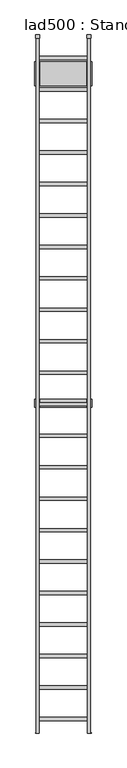
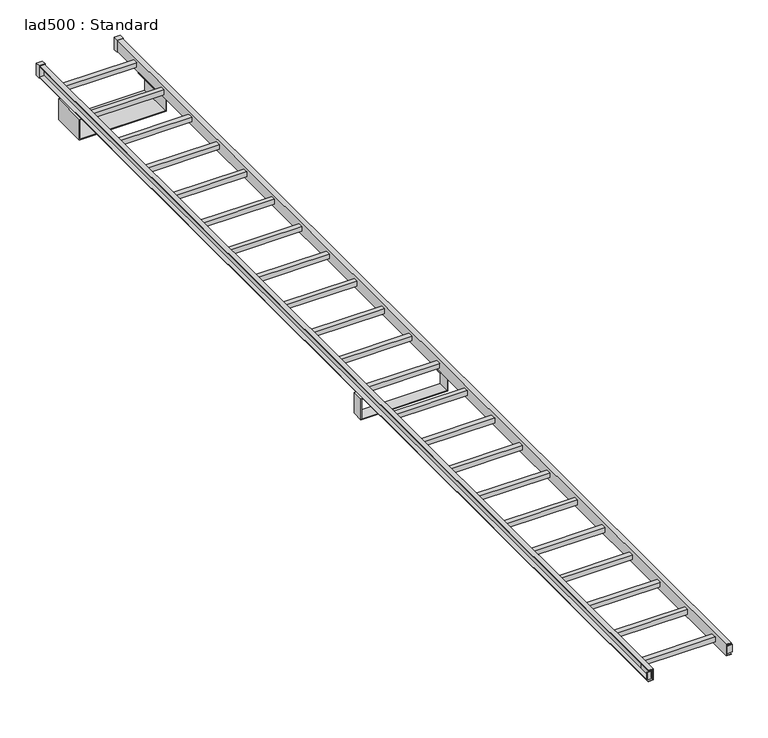
"""IFC4 building model written with IfcOpenShell, lengths in millimetres: proxy geometry, lad500 : Standard."""

from ifc_helpers import new_model, si_unit, point, frame, frame_2d, origin, place, context, project, spatial, polyline, circle_curve, trimmed, segment, composite_curve, outline, extrude, source, transform, mapped, element, save


def lad500_standard_3a90afe1(model_context):
    return source(origin(), model_context, "Body", "SweptSolid", [
        extrude(outline(polyline([(-233.3625, -1309.5859108), (-233.3625, -1277.8359108), (233.3625, -1277.8359108), (233.3625, -1309.5859108), (-233.3625, -1309.5859108)])), frame((0.0, 0.0, 161.925), z_axis=(0.0, 0.0, 1.0), x_axis=(1.0, 0.0, 0.0)), (0.0, 0.0, 1.0), 31.75),
        extrude(outline(polyline([(-233.3625, -1004.7859108), (-233.3625, -973.0359108), (233.3625, -973.0359108), (233.3625, -1004.7859108), (-233.3625, -1004.7859108)])), frame((0.0, 0.0, 161.925), z_axis=(0.0, 0.0, 1.0), x_axis=(1.0, 0.0, 0.0)), (0.0, 0.0, 1.0), 31.75),
        extrude(outline(polyline([(-233.3625, -699.9859108), (-233.3625, -668.2359108), (233.3625, -668.2359108), (233.3625, -699.9859108), (-233.3625, -699.9859108)])), frame((0.0, 0.0, 161.925), z_axis=(0.0, 0.0, 1.0), x_axis=(1.0, 0.0, 0.0)), (0.0, 0.0, 1.0), 31.75),
        extrude(outline(polyline([(-233.3625, -395.1859108), (-233.3625, -363.4359108), (233.3625, -363.4359108), (233.3625, -395.1859108), (-233.3625, -395.1859108)])), frame((0.0, 0.0, 161.925), z_axis=(0.0, 0.0, 1.0), x_axis=(1.0, 0.0, 0.0)), (0.0, 0.0, 1.0), 31.75),
        extrude(outline(polyline([(-233.3625, -90.3859108), (-233.3625, -58.6359108), (233.3625, -58.6359108), (233.3625, -90.3859108), (-233.3625, -90.3859108)])), frame((0.0, 0.0, 161.925), z_axis=(0.0, 0.0, 1.0), x_axis=(1.0, 0.0, 0.0)), (0.0, 0.0, 1.0), 31.75),
        extrude(outline(polyline([(-233.3625, 214.4140892), (-233.3625, 246.1640892), (233.3625, 246.1640892), (233.3625, 214.4140892), (-233.3625, 214.4140892)])), frame((0.0, 0.0, 161.925), z_axis=(0.0, 0.0, 1.0), x_axis=(1.0, 0.0, 0.0)), (0.0, 0.0, 1.0), 31.75),
        extrude(outline(polyline([(-233.3625, 519.2140892), (-233.3625, 550.9640892), (233.3625, 550.9640892), (233.3625, 519.2140892), (-233.3625, 519.2140892)])), frame((0.0, 0.0, 161.925), z_axis=(0.0, 0.0, 1.0), x_axis=(1.0, 0.0, 0.0)), (0.0, 0.0, 1.0), 31.75),
        extrude(outline(polyline([(-233.3625, 824.0140892), (-233.3625, 855.7640892), (233.3625, 855.7640892), (233.3625, 824.0140892), (-233.3625, 824.0140892)])), frame((0.0, 0.0, 161.925), z_axis=(0.0, 0.0, 1.0), x_axis=(1.0, 0.0, 0.0)), (0.0, 0.0, 1.0), 31.75),
        extrude(outline(polyline([(-233.3625, 1128.8140892), (-233.3625, 1160.5640892), (233.3625, 1160.5640892), (233.3625, 1128.8140892), (-233.3625, 1128.8140892)])), frame((0.0, 0.0, 161.925), z_axis=(0.0, 0.0, 1.0), x_axis=(1.0, 0.0, 0.0)), (0.0, 0.0, 1.0), 31.75),
        extrude(outline(polyline([(-233.3625, 1433.6140892), (-233.3625, 1465.3640892), (233.3625, 1465.3640892), (233.3625, 1433.6140892), (-233.3625, 1433.6140892)])), frame((0.0, 0.0, 161.925), z_axis=(0.0, 0.0, 1.0), x_axis=(1.0, 0.0, 0.0)), (0.0, 0.0, 1.0), 31.75),
        extrude(outline(polyline([(-233.3625, 1738.4140892), (-233.3625, 1770.1640892), (233.3625, 1770.1640892), (233.3625, 1738.4140892), (-233.3625, 1738.4140892)])), frame((0.0, 0.0, 161.925), z_axis=(0.0, 0.0, 1.0), x_axis=(1.0, 0.0, 0.0)), (0.0, 0.0, 1.0), 31.75),
        extrude(outline(polyline([(-233.3625, 2043.2140892), (-233.3625, 2074.9640892), (233.3625, 2074.9640892), (233.3625, 2043.2140892), (-233.3625, 2043.2140892)])), frame((0.0, 0.0, 161.925), z_axis=(0.0, 0.0, 1.0), x_axis=(1.0, 0.0, 0.0)), (0.0, 0.0, 1.0), 31.75),
        extrude(outline(polyline([(-233.3625, 2348.0140892), (-233.3625, 2379.7640892), (233.3625, 2379.7640892), (233.3625, 2348.0140892), (-233.3625, 2348.0140892)])), frame((0.0, 0.0, 161.925), z_axis=(0.0, 0.0, 1.0), x_axis=(1.0, 0.0, 0.0)), (0.0, 0.0, 1.0), 31.75),
        extrude(outline(polyline([(-233.3625, 2652.8140892), (-233.3625, 2684.5640892), (233.3625, 2684.5640892), (233.3625, 2652.8140892), (-233.3625, 2652.8140892)])), frame((0.0, 0.0, 161.925), z_axis=(0.0, 0.0, 1.0), x_axis=(1.0, 0.0, 0.0)), (0.0, 0.0, 1.0), 31.75),
        extrude(outline(polyline([(-233.3625, 2957.6140892), (-233.3625, 2989.3640892), (233.3625, 2989.3640892), (233.3625, 2957.6140892), (-233.3625, 2957.6140892)])), frame((0.0, 0.0, 161.925), z_axis=(0.0, 0.0, 1.0), x_axis=(1.0, 0.0, 0.0)), (0.0, 0.0, 1.0), 31.75),
        extrude(outline(polyline([(-233.3625, 3262.4140892), (-233.3625, 3294.1640892), (233.3625, 3294.1640892), (233.3625, 3262.4140892), (-233.3625, 3262.4140892)])), frame((0.0, 0.0, 161.925), z_axis=(0.0, 0.0, 1.0), x_axis=(1.0, 0.0, 0.0)), (0.0, 0.0, 1.0), 31.75),
        extrude(outline(polyline([(-233.3625, 3567.2140892), (-233.3625, 3598.9640892), (233.3625, 3598.9640892), (233.3625, 3567.2140892), (-233.3625, 3567.2140892)])), frame((0.0, 0.0, 161.925), z_axis=(0.0, 0.0, 1.0), x_axis=(1.0, 0.0, 0.0)), (0.0, 0.0, 1.0), 31.75),
        extrude(outline(polyline([(-233.3625, 3872.0140892), (-233.3625, 3903.7640892), (233.3625, 3903.7640892), (233.3625, 3872.0140892), (-233.3625, 3872.0140892)])), frame((0.0, 0.0, 161.925), z_axis=(0.0, 0.0, 1.0), x_axis=(1.0, 0.0, 0.0)), (0.0, 0.0, 1.0), 31.75),
        extrude(outline(polyline([(-233.3625, 4176.8140892), (-233.3625, 4208.5640892), (233.3625, 4208.5640892), (233.3625, 4176.8140892), (-233.3625, 4176.8140892)])), frame((0.0, 0.0, 161.925), z_axis=(0.0, 0.0, 1.0), x_axis=(1.0, 0.0, 0.0)), (0.0, 0.0, 1.0), 31.75),
        extrude(outline(polyline([(-233.3625, 4481.6140892), (-233.3625, 4513.3640892), (233.3625, 4513.3640892), (233.3625, 4481.6140892), (-233.3625, 4481.6140892)])), frame((0.0, 0.0, 161.925), z_axis=(0.0, 0.0, 1.0), x_axis=(1.0, 0.0, 0.0)), (0.0, 0.0, 1.0), 31.75),
        extrude(outline(polyline([(-233.3625, 4786.4140892), (-233.3625, 4818.1640892), (233.3625, 4818.1640892), (233.3625, 4786.4140892), (-233.3625, 4786.4140892)])), frame((0.0, 0.0, 161.925), z_axis=(0.0, 0.0, 1.0), x_axis=(1.0, 0.0, 0.0)), (0.0, 0.0, 1.0), 31.75),
        extrude(outline(polyline([(-233.3625, 5091.2140892), (-233.3625, 5122.9640892), (233.3625, 5122.9640892), (233.3625, 5091.2140892), (-233.3625, 5091.2140892)])), frame((0.0, 0.0, 161.925), z_axis=(0.0, 0.0, 1.0), x_axis=(1.0, 0.0, 0.0)), (0.0, 0.0, 1.0), 31.75),
        extrude(outline(polyline([(139.7, -230.1875), (139.7, -277.8125), (0.0, -277.8125), (0.0, 277.8125), (139.7, 277.8125), (139.7, 230.1875), (134.9375, 230.1875), (134.9375, 273.05), (4.7625, 273.05), (4.7625, -273.05), (134.9375, -273.05), (134.9375, -230.1875), (139.7, -230.1875)])), frame((0.0, 1724.1265892, 0.0), z_axis=(0.0, 1.0, 0.0), x_axis=(0.0, 0.0, 1.0)), (0.0, 0.0, 1.0), 76.2),
        extrude(outline(polyline([(139.7, -230.1875), (139.7, -277.8125), (0.0, -277.8125), (0.0, 277.8125), (139.7, 277.8125), (139.7, 230.1875), (134.9375, 230.1875), (134.9375, 273.05), (4.7625, 273.05), (4.7625, -273.05), (134.9375, -273.05), (134.9375, -230.1875), (139.7, -230.1875)])), frame((0.0, 4840.3890892, 0.0), z_axis=(0.0, 1.0, 0.0), x_axis=(0.0, 0.0, 1.0)), (0.0, 0.0, 1.0), 228.6),
        extrude(outline(polyline([(215.9, 265.1125), (215.9, 233.3625), (139.7, 233.3625), (139.7, 265.1125), (142.875, 265.1125), (142.875, 236.5375), (212.725, 236.5375), (212.725, 265.1125), (215.9, 265.1125)])), frame((0.0, -1430.2359108, 0.0), z_axis=(0.0, 1.0, 0.0), x_axis=(0.0, 0.0, 1.0)), (0.0, 0.0, 1.0), 6756.4),
        extrude(outline(polyline([(215.9, -265.1125), (212.725, -265.1125), (212.725, -236.5375), (142.875, -236.5375), (142.875, -265.1125), (139.7, -265.1125), (139.7, -233.3625), (215.9, -233.3625), (215.9, -265.1125)])), frame((0.0, -1430.2359108, 0.0), z_axis=(0.0, 1.0, 0.0), x_axis=(0.0, 0.0, 1.0)), (0.0, 0.0, 1.0), 6756.4),
        extrude(outline(polyline([(230.1875, 5330.9265892), (268.2875, 5330.9265892), (268.2875, 5300.7640892), (230.1875, 5300.7640892), (230.1875, 5330.9265892)])), frame((0.0, 0.0, 136.525), z_axis=(0.0, 0.0, 1.0), x_axis=(1.0, 0.0, 0.0)), (0.0, 0.0, 1.0), 82.55),
        extrude(outline(polyline([(-268.2875, 5330.9265892), (-230.1875, 5330.9265892), (-230.1875, 5300.7640892), (-268.2875, 5300.7640892), (-268.2875, 5330.9265892)])), frame((0.0, 0.0, 136.525), z_axis=(0.0, 0.0, 1.0), x_axis=(1.0, 0.0, 0.0)), (0.0, 0.0, 1.0), 82.55),
        extrude(outline(composite_curve([segment(polyline([(236.5375, -1430.2359108), (236.5375, -1315.9359108), (241.3, -1315.9359108), (241.3, -1422.2984108)]), True, "CONTINUOUS"), segment(trimmed(circle_curve(frame_2d((244.475, -1422.2984108)), 3.175), [point((241.3, -1422.2984108))], [point((244.475, -1425.4734108))], True, "CARTESIAN"), True, "CONTINUOUS"), segment(polyline([(244.475, -1425.4734108), (271.4625, -1425.4734108), (271.4625, -1430.2359108), (236.5375, -1430.2359108)]), True, "CONTINUOUS")], self_intersect=False)), frame((0.0, 0.0, 152.4), z_axis=(0.0, 0.0, 1.0), x_axis=(1.0, 0.0, 0.0)), (0.0, 0.0, 1.0), 50.8),
        extrude(outline(composite_curve([segment(polyline([(-236.5375, -1430.2359108), (-271.4625, -1430.2359108), (-271.4625, -1425.4734108), (-244.475, -1425.4734108)]), True, "CONTINUOUS"), segment(trimmed(circle_curve(frame_2d((-244.475, -1422.2984108)), 3.175), [point((-244.475, -1425.4734108))], [point((-241.3, -1422.2984108))], True, "CARTESIAN"), True, "CONTINUOUS"), segment(polyline([(-241.3, -1422.2984108), (-241.3, -1315.9359108), (-236.5375, -1315.9359108), (-236.5375, -1430.2359108)]), True, "CONTINUOUS")], self_intersect=False)), frame((0.0, 0.0, 152.4), z_axis=(0.0, 0.0, 1.0), x_axis=(1.0, 0.0, 0.0)), (0.0, 0.0, 1.0), 50.8),
    ])


if __name__ == "__main__":
    model = new_model("IFC4")
    model_context = context("Model", 3, world=origin())
    ifc_project = project(units=[si_unit("LENGTHUNIT", "METRE", prefix="MILLI")], contexts=[model_context])
    site = spatial("IfcSite", under=ifc_project)
    building = spatial("IfcBuilding", under=site)
    placement = place(None, origin())
    lad500_standard_shape = lad500_standard_3a90afe1(model_context)
    element("IfcBuildingElementProxy", 1, Name="lad500 : Standard", ObjectType="lad500 : Standard", at=placement, inside=building, context=model_context, shape_type="MappedRepresentation", body=[
        mapped(lad500_standard_shape, transform((0.0, 0.0, 0.0), x_axis=(1.0, 0.0, 0.0), y_axis=(0.0, 1.0, 0.0), z_axis=(0.0, 0.0, 1.0))),
    ])
    save(model, "model.ifc")

# Revit data of these elements
# Type "lad500 : Standard"
#   Version = "1"
#   URL = "http://www.okeeffes.com/"
#   Series = "Access Ladders"
#   Product Page URL = "http://www.okeeffes.com/ladders/details/lad500.pdf"
#   Model = "500"
#   Manufacturer = "O'Keeffe's, Inc."
#   Description = "Standard Duty Channel Rail - Fixed Access Aluminum Ladder"
#   Assembly Code = "B1010700"
#   Wall To Center Line Of Ladder [instance default] = 0' - 7"
#   Top of Decking [instance default] = 10' - 3 1/2"
#   Top Support Offset from Decking [instance default] = 0' - 6 5/8"
#   Roof Hatch Base Height [instance default] = 1' - 0"
#   Overall Width [instance default] = 1' - 9 7/8"
#   Overall Length [instance default] = 0' - 8 1/2"
#   Overall Height [instance default] = 10' - 11 1/2"
#   Bottom Support Offset from Floor [instance default] = 1' - 4"
#   Middle Support Offset from Floor [instance default] = 4' - 10 7/16"
#   Off Floor Clearance [instance default] = 0' - 0"
#   Ladder Width [instance default] = 1' - 6 3/8"
#   With Roof Hatch [instance default] = no
#   Rungs Quantity Control [instance default] = 11
#   Rungs Quantity [instance default] = 10
#   On Floor Support [instance default] = yes
#   Off Floor Support [instance default] = no
#   Ladder Material = PREFABRICATED METAL SHIPS LADDER
#   Default Elevation = 0
# Element 1 (IfcBuildingElementProxy, "lad500 : Standard")
#   Top of Decking = 21' - 6"
#   Overall Height = 22' - 2"
#   Middle Support Offset from Floor = 10' - 5 11/16"
#   Rungs Quantity Control = 22
#   Rungs Quantity = 22
#   Materials on its faces: "PREFABRICATED METAL SHIPS LADDER"
# Materials
#   "PREFABRICATED METAL SHIPS LADDER": class "Metal", colour RGB 192 192 192, transparency 0, Cost = 0
